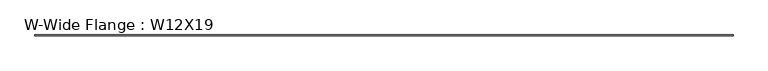
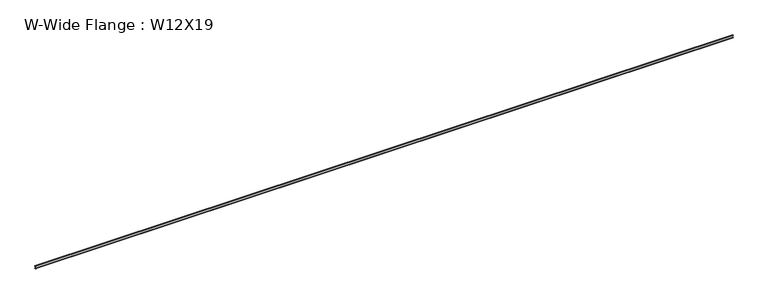
"""IFC4 building model written with IfcOpenShell, lengths in millimetres: beam geometry, W-Wide Flange : W12X19."""

import ifcopenshell
import ifcopenshell.guid

model = None  # the IFC model being written
_history = None  # IfcOwnerHistory: only IFC2X3 demands one
_inside = {}  # id of a spatial element -> (the spatial element, [elements in it])
_under = {}  # id of a project, library or spatial element -> (it, [spatial elements below it])
_declared = {}  # id of a project -> (the project, [libraries it declares])
_typed = {}  # id of a type object -> (the type object, [elements of that type])
_made_of = {}  # id of a material, layer set ... -> (it, [elements and type objects made of it])


def new_model(schema):
    """Start an empty IFC model of exactly this schema.

    Asked for "IFC4X3", IfcOpenShell would pick the latest addendum, in which some entities
    have other attributes; the version numbers below select the first issue.
    IFC2X3 requires an IfcOwnerHistory on every rooted entity: one is made here for all.
    """
    global model, _history
    if schema == "IFC4X3":
        model = ifcopenshell.file(schema_version=(4, 3, 0, 0))
    else:
        model = ifcopenshell.file(schema=schema)
    _inside.clear()
    _under.clear()
    _declared.clear()
    _typed.clear()
    _made_of.clear()
    _history = None
    if model.schema == "IFC2X3":
        org = make("IfcOrganization", Name="unknown")
        user = make(
            "IfcPersonAndOrganization",
            ThePerson=make("IfcPerson", FamilyName="unknown"),
            TheOrganization=org,
        )
        app = make(
            "IfcApplication",
            ApplicationDeveloper=org,
            Version="unknown",
            ApplicationFullName="unknown",
            ApplicationIdentifier="unknown",
        )
        _history = make(
            "IfcOwnerHistory",
            OwningUser=user,
            OwningApplication=app,
            ChangeAction="ADDED",
            CreationDate=0,
        )
    return model


def make(cls, **values):
    """One entity of the class cls with the attributes given. An attribute that is None is left unset."""
    return model.create_entity(
        cls, **{name: value for name, value in values.items() if value is not None}
    )


def rooted(cls, **values):
    """An entity with a GlobalId (a new one), such as an element, a storey or a relation."""
    return make(cls, GlobalId=ifcopenshell.guid.new(), OwnerHistory=_history, **values)


def si_unit(unit_type, name, prefix=None):
    """IfcSIUnit, for example si_unit("LENGTHUNIT", "METRE", prefix="MILLI")."""
    return make("IfcSIUnit", UnitType=unit_type, Prefix=prefix, Name=name)


def assignment(units):
    """IfcUnitAssignment: the units of a project."""
    return None if units is None else make("IfcUnitAssignment", Units=units)


def point(xyz):
    """IfcCartesianPoint."""
    return None if xyz is None else make("IfcCartesianPoint", Coordinates=xyz)


def direction(xyz):
    """IfcDirection."""
    return None if xyz is None else make("IfcDirection", DirectionRatios=xyz)


def frame(location, z_axis=None, x_axis=None):
    """IfcAxis2Placement3D, a coordinate frame: its origin and axes. An axis left out is left unset."""
    return make(
        "IfcAxis2Placement3D",
        Location=point(location),
        Axis=direction(z_axis),
        RefDirection=direction(x_axis),
    )


def frame_2d(location, x_axis=None):
    """IfcAxis2Placement2D, a coordinate frame in the plane: its origin and x axis."""
    return make(
        "IfcAxis2Placement2D", Location=point(location), RefDirection=direction(x_axis)
    )


def origin():
    """The frame at (0, 0, 0) with its axes left unset."""
    return frame((0.0, 0.0, 0.0))


def place(relative_to, where):
    """IfcLocalPlacement: puts the frame where relative to a parent placement (None: the world)."""
    return make(
        "IfcLocalPlacement", PlacementRelTo=relative_to, RelativePlacement=where
    )


def context(
    kind, dimensions, precision=None, world=None, true_north=None, identifier=None
):
    """IfcGeometricRepresentationContext, for example the 3D "Model" context."""
    return make(
        "IfcGeometricRepresentationContext",
        ContextIdentifier=identifier,
        ContextType=kind,
        CoordinateSpaceDimension=dimensions,
        Precision=precision,
        WorldCoordinateSystem=world,
        TrueNorth=true_north,
    )


def project(units=None, contexts=None):
    """IfcProject with its units and contexts."""
    return rooted(
        "IfcProject",
        Name="project",
        RepresentationContexts=contexts,
        UnitsInContext=assignment(units),
    )


def spatial(cls, under=None, at=None, **own):
    """A site, building, storey or space (cls), placed at a placement, below another one or the project."""
    s = rooted(cls, ObjectPlacement=at, **own)
    if under is not None:
        _under.setdefault(under.id(), (under, []))[1].append(s)
    return s


def polyline(points):
    """IfcPolyline through the points."""
    return make("IfcPolyline", Points=[point(p) for p in points])


def circle_curve(where, radius):
    """IfcCircle in the frame where."""
    return make("IfcCircle", Position=where, Radius=radius)


def trimmed(basis, trim1, trim2, sense, master):
    """IfcTrimmedCurve: the piece of a basis curve between two trims."""
    return make(
        "IfcTrimmedCurve",
        BasisCurve=basis,
        Trim1=trim1,
        Trim2=trim2,
        SenseAgreement=sense,
        MasterRepresentation=master,
    )


def segment(curve, same_sense, transition):
    """IfcCompositeCurveSegment."""
    return make(
        "IfcCompositeCurveSegment",
        Transition=transition,
        SameSense=same_sense,
        ParentCurve=curve,
    )


def composite_curve(segments, self_intersect=None):
    """IfcCompositeCurve: segments joined end to end."""
    return make("IfcCompositeCurve", Segments=segments, SelfIntersect=self_intersect)


def outline(outer, holes=None, kind="AREA"):
    """IfcArbitraryClosedProfileDef: a profile drawn as a closed curve; with holes, ...WithVoids."""
    if holes is None:
        return make("IfcArbitraryClosedProfileDef", ProfileType=kind, OuterCurve=outer)
    return make(
        "IfcArbitraryProfileDefWithVoids",
        ProfileType=kind,
        OuterCurve=outer,
        InnerCurves=holes,
    )


def extrude(swept, where, along, depth):
    """IfcExtrudedAreaSolid: the profile swept, set in the frame where, extruded along a direction by depth."""
    return make(
        "IfcExtrudedAreaSolid",
        SweptArea=swept,
        Position=where,
        ExtrudedDirection=direction(along),
        Depth=depth,
    )


def shape(context_of_items, identifier, shape_type, items):
    """IfcShapeRepresentation: the items that make up one representation, for example the "Body"."""
    return make(
        "IfcShapeRepresentation",
        ContextOfItems=context_of_items,
        RepresentationIdentifier=identifier,
        RepresentationType=shape_type,
        Items=items,
    )


def source(mapping_origin, context_of_items, identifier, shape_type, items):
    """IfcRepresentationMap: a shape defined once, which mapped items show again and again."""
    return make(
        "IfcRepresentationMap",
        MappingOrigin=mapping_origin,
        MappedRepresentation=shape(context_of_items, identifier, shape_type, items),
    )


def transform(
    local_origin,
    x_axis=None,
    y_axis=None,
    z_axis=None,
    scale=None,
    scale2=None,
    scale3=None,
    uniform=True,
):
    """IfcCartesianTransformationOperator3D, or its non-uniform kind. x_axis, y_axis, z_axis: its Axis1, 2, 3."""
    if uniform:
        return make(
            "IfcCartesianTransformationOperator3D",
            Axis1=direction(x_axis),
            Axis2=direction(y_axis),
            LocalOrigin=point(local_origin),
            Scale=scale,
            Axis3=direction(z_axis),
        )
    return make(
        "IfcCartesianTransformationOperator3DnonUniform",
        Axis1=direction(x_axis),
        Axis2=direction(y_axis),
        LocalOrigin=point(local_origin),
        Scale=scale,
        Axis3=direction(z_axis),
        Scale2=scale2,
        Scale3=scale3,
    )


def mapped(mapping_source, mapping_target):
    """IfcMappedItem: shows the shape of a source again, moved by a transform."""
    return make(
        "IfcMappedItem", MappingSource=mapping_source, MappingTarget=mapping_target
    )


def made_of(thing, what):
    """Note that an element or type object is made of a material, layer set ...; save() writes the relation."""
    if what is not None:
        _made_of.setdefault(what.id(), (what, []))[1].append(thing)
    return thing


def element(
    cls,
    number,
    at=None,
    inside=None,
    cuts=None,
    type_object=None,
    material=None,
    context=None,
    identifier="Body",
    shape_type=None,
    held_by="IfcProductDefinitionShape",
    body=None,
    shapes=None,
    **own,
):
    """One element of the class cls, such as IfcWall. Its Tag is "e" and its number.

    at: its placement. inside: the storey or other place that contains it. cuts: it is an
    opening in that element (IfcRelVoidsElement). A single representation is given by context,
    identifier, shape_type and body (its items); several are given by shapes. held_by: the class
    of the entity that holds the representations. save() writes the other relations.
    """
    e = rooted(cls, Tag="e%d" % number, ObjectPlacement=at, **own)
    if body is not None:
        shapes = [shape(context, identifier, shape_type, body)]
    if shapes is not None:
        e.Representation = make(held_by, Representations=shapes)
    if inside is not None:
        _inside.setdefault(inside.id(), (inside, []))[1].append(e)
    if cuts is not None:
        rooted(
            "IfcRelVoidsElement", RelatingBuildingElement=cuts, RelatedOpeningElement=e
        )
    if type_object is not None:
        _typed.setdefault(type_object.id(), (type_object, []))[1].append(e)
    return made_of(e, material)


def aggregate(whole, parts):
    """IfcRelAggregates: a whole, such as a stair, and the parts it consists of."""
    return rooted("IfcRelAggregates", RelatingObject=whole, RelatedObjects=parts)


def save(model, path):
    """Write the relations noted so far, then the file.

    IfcRelAggregates (storeys below a building ...), IfcRelContainedInSpatialStructure (elements
    in a storey), IfcRelDefinesByType, IfcRelAssociatesMaterial and IfcRelDeclares: one each for
    every whole, place, type object, material and project.
    """
    for whole, parts in _under.values():
        aggregate(whole, parts)
    for where, things in _inside.values():
        rooted(
            "IfcRelContainedInSpatialStructure",
            RelatedElements=things,
            RelatingStructure=where,
        )
    for kind, things in _typed.values():
        rooted("IfcRelDefinesByType", RelatedObjects=things, RelatingType=kind)
    for what, things in _made_of.values():
        rooted("IfcRelAssociatesMaterial", RelatedObjects=things, RelatingMaterial=what)
    for by, libraries in _declared.values():
        rooted("IfcRelDeclares", RelatingContext=by, RelatedDefinitions=libraries)
    model.write(path)


def w_wide_flange_w12x19_a1d3db04(model_context):
    return source(origin(), model_context, "Body", "SweptSolid", [
        extrude(outline(composite_curve([segment(polyline([(50.927, -146.05), (50.927, -154.94), (-50.927, -154.94), (-50.927, -146.05), (-16.3195, -146.05)]), True, "CONTINUOUS"), segment(trimmed(circle_curve(frame_2d((-16.3195, -132.715)), 13.335), [point((-16.3195, -146.05))], [point((-2.9845, -132.715))], True, "CARTESIAN"), True, "CONTINUOUS"), segment(polyline([(-2.9845, -132.715), (-2.9845, 132.715)]), True, "CONTINUOUS"), segment(trimmed(circle_curve(frame_2d((-16.3195, 132.715)), 13.335), [point((-2.9845, 132.715))], [point((-16.3195, 146.05))], True, "CARTESIAN"), True, "CONTINUOUS"), segment(polyline([(-16.3195, 146.05), (-50.927, 146.05), (-50.927, 154.94), (50.927, 154.94), (50.927, 146.05), (16.3195, 146.05)]), True, "CONTINUOUS"), segment(trimmed(circle_curve(frame_2d((16.3195, 132.715)), 13.335), [point((16.3195, 146.05))], [point((2.9845, 132.715))], True, "CARTESIAN"), True, "CONTINUOUS"), segment(polyline([(2.9845, 132.715), (2.9845, -132.715)]), True, "CONTINUOUS"), segment(trimmed(circle_curve(frame_2d((16.3195, -132.715)), 13.335), [point((2.9845, -132.715))], [point((16.3195, -146.05))], True, "CARTESIAN"), True, "CONTINUOUS"), segment(polyline([(16.3195, -146.05), (50.927, -146.05)]), True, "CONTINUOUS")], self_intersect=False)), frame((-43980.1, 0.0, 0.0), z_axis=(1.0, 0.0, 0.0), x_axis=(0.0, 1.0, 0.0)), (0.0, 0.0, 1.0), 88011.0),
    ])


if __name__ == "__main__":
    model = new_model("IFC4")
    model_context = context("Model", 3, world=origin())
    ifc_project = project(units=[si_unit("LENGTHUNIT", "METRE", prefix="MILLI")], contexts=[model_context])
    site = spatial("IfcSite", under=ifc_project)
    building = spatial("IfcBuilding", under=site)
    placement = place(None, origin())
    w_wide_flange_w12x19_shape = w_wide_flange_w12x19_a1d3db04(model_context)
    element("IfcBeam", 1, ObjectType="W-Wide Flange : W12X19", at=placement, inside=building, context=model_context, shape_type="MappedRepresentation", body=[
        mapped(w_wide_flange_w12x19_shape, transform((0.0, 0.0, 0.0), x_axis=(1.0, 0.0, 0.0), y_axis=(0.0, 1.0, 0.0), z_axis=(0.0, 0.0, 1.0))),
    ])
    save(model, "model.ifc")

# Revit data of these elements
# Type "W-Wide Flange : W12X19"
#   Assembly Code = "B10"
#   W = 19
#   Length [instance default] = 5' - 0"
#   bf = 0' - 4.01"
#   d = 1' - 0.2"
#   k = 0' - 0 7/8"
#   k2 = 0' - 0.525"
#   tf = 0' - 0.35"
#   tw = 0' - 0.235"
#   A = 0.0386806 SF
#   Structural Material [instance default] = Steel ASTM A992
# Element 1 (IfcBeam, "W-Wide Flange : W12X19")
#   Structural Material = STRUCTURAL STEEL - SEE STRUCT. DWGS
#   Materials on its faces: "STRUCTURAL STEEL - SEE STRUCT. DWGS"
# Materials
#   "Steel ASTM A992": class "Metal", colour RGB 199 199 199, transparency 0, Description = "Structural steel 50ksi", Cost = 0
#   "STRUCTURAL STEEL - SEE STRUCT. DWGS": class "Metal", colour RGB 137 146 153, transparency 0, Description = "Steel, mill finish", Cost = 0
